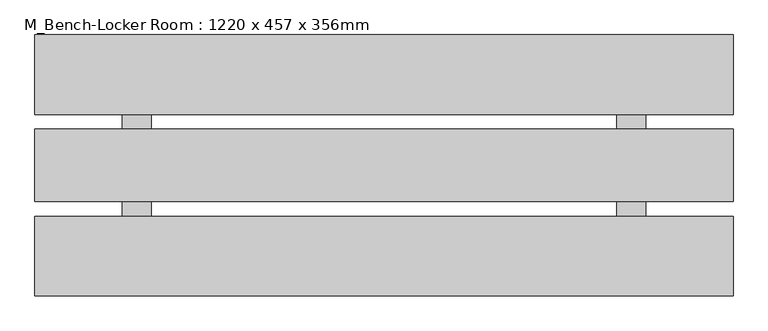
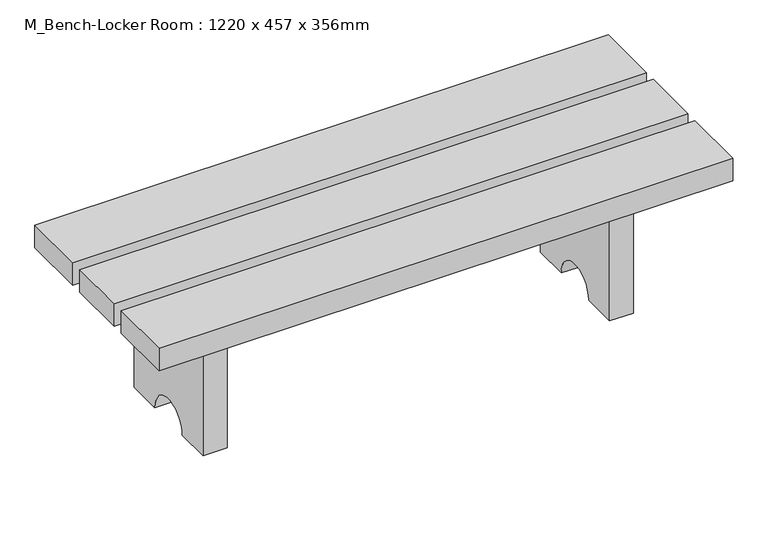
"""IFC4 building model written with IfcOpenShell, lengths in millimetres: furniture geometry, M_Bench-Locker Room : 1220 x 457 x 356mm."""

from ifc_helpers import new_model, si_unit, point, frame, frame_2d, origin, place, context, project, spatial, polyline, circle_curve, trimmed, segment, composite_curve, outline, extrude, source, transform, mapped, element, save


def m_bench_locker_room_1220_x_457_x_356mm_e5efdec1(model_context):
    return source(origin(), model_context, "Body", "SweptSolid", [
        extrude(outline(composite_curve([segment(polyline([(307.6147541, 0.0), (231.4147541, 0.0)]), True, "CONTINUOUS"), segment(trimmed(circle_curve(frame_2d((180.7147541, 0.0)), 50.7), [point((231.4147541, 0.0))], [point((130.0147541, 0.0))], True, "CARTESIAN"), True, "CONTINUOUS"), segment(polyline([(130.0147541, 0.0), (53.8147541, 0.0), (53.8147541, 305.2), (307.6147541, 305.2), (307.6147541, 0.0)]), True, "CONTINUOUS")], self_intersect=False)), frame((251.4852459, 0.0, 0.0), z_axis=(1.0, 0.0, 0.0), x_axis=(0.0, 1.0, 0.0)), (0.0, 0.0, 1.0), 50.8),
        extrude(outline(composite_curve([segment(polyline([(53.8147541, 0.0), (53.8147541, 305.2), (307.6147541, 305.2), (307.6147541, 0.0), (231.4147541, 0.0)]), True, "CONTINUOUS"), segment(trimmed(circle_curve(frame_2d((180.7147541, 0.0)), 50.7), [point((231.4147541, 0.0))], [point((130.0147541, 0.0))], True, "CARTESIAN"), True, "CONTINUOUS"), segment(polyline([(130.0147541, 0.0), (53.8147541, 0.0)]), True, "CONTINUOUS")], self_intersect=False)), frame((-612.9147541, 0.0, 0.0), z_axis=(1.0, 0.0, 0.0), x_axis=(0.0, 1.0, 0.0)), (0.0, 0.0, 1.0), 50.8),
        extrude(outline(polyline([(454.6852459, -47.7852459), (-765.3147541, -47.7852459), (-765.3147541, 91.8480874), (454.6852459, 91.8480874), (454.6852459, -47.7852459)])), frame((0.0, 0.0, 305.2), z_axis=(0.0, 0.0, 1.0), x_axis=(1.0, 0.0, 0.0)), (0.0, 0.0, 1.0), 50.8),
        extrude(outline(polyline([(454.6852459, 409.2147541), (454.6852459, 269.5814208), (-765.3147541, 269.5814208), (-765.3147541, 409.2147541), (454.6852459, 409.2147541)])), frame((0.0, 0.0, 305.2), z_axis=(0.0, 0.0, 1.0), x_axis=(1.0, 0.0, 0.0)), (0.0, 0.0, 1.0), 50.8),
        extrude(outline(polyline([(454.6852459, 117.2480874), (-765.3147541, 117.2480874), (-765.3147541, 244.1814208), (454.6852459, 244.1814208), (454.6852459, 117.2480874)])), frame((0.0, 0.0, 305.2), z_axis=(0.0, 0.0, 1.0), x_axis=(1.0, 0.0, 0.0)), (0.0, 0.0, 1.0), 50.8),
    ])


if __name__ == "__main__":
    model = new_model("IFC4")
    model_context = context("Model", 3, world=origin())
    ifc_project = project(units=[si_unit("LENGTHUNIT", "METRE", prefix="MILLI")], contexts=[model_context])
    site = spatial("IfcSite", under=ifc_project)
    building = spatial("IfcBuilding", under=site)
    placement = place(None, origin())
    m_bench_locker_room_1220_x_457_x_356mm_shape = m_bench_locker_room_1220_x_457_x_356mm_e5efdec1(model_context)
    element("IfcFurniture", 1, ObjectType="M_Bench-Locker Room : 1220 x 457 x 356mm", at=placement, inside=building, context=model_context, shape_type="MappedRepresentation", body=[
        mapped(m_bench_locker_room_1220_x_457_x_356mm_shape, transform((0.0, 0.0, 0.0), x_axis=(1.0, 0.0, 0.0), y_axis=(0.0, 1.0, 0.0), z_axis=(0.0, 0.0, 1.0))),
    ])
    save(model, "model.ifc")

# Revit data of these elements
# Type "M_Bench-Locker Room : 1220 x 457 x 356mm"
#   Depth = 0.457 m
#   Height = 0.356 m
#   Width = 1.22 m
#   Bench Material = Cherry
#   Default Elevation = 0
# Element 1 (IfcFurniture, "M_Bench-Locker Room : 1220 x 457 x 356mm")
#   Materials on its faces: "Cherry"
# Materials
#   "Cherry": class "Wood", colour RGB 226 177 128, transparency 0, Description = "Prunus Serotina", Cost = 0
